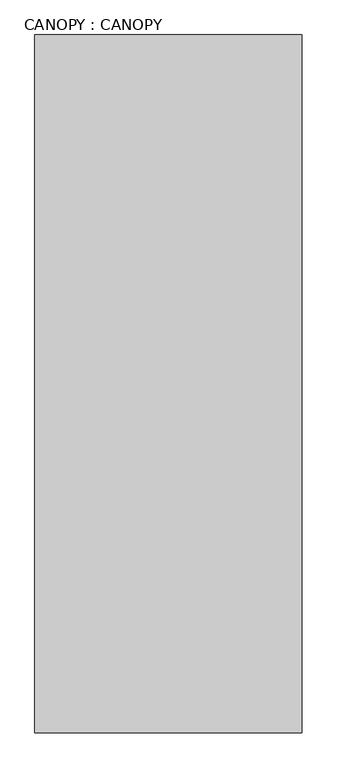
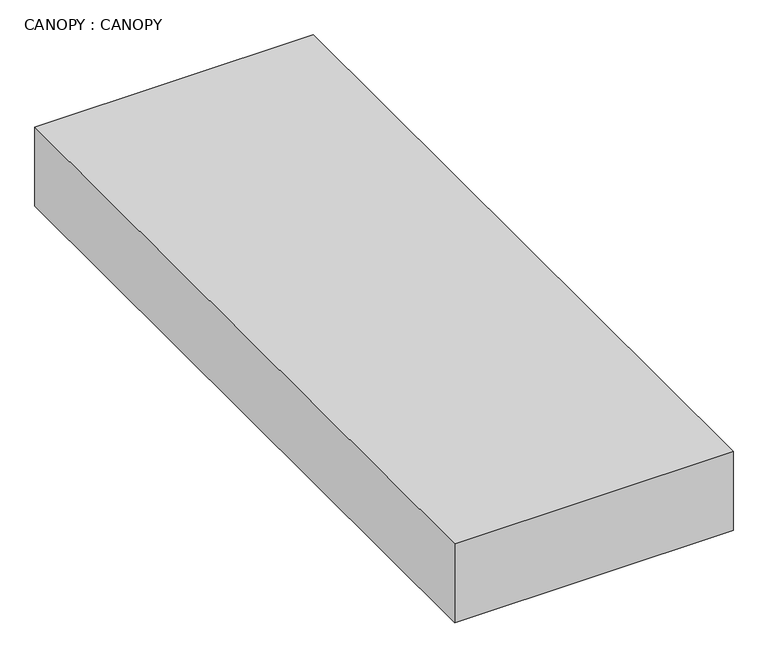
"""IFC4 building model written with IfcOpenShell, lengths in millimetres: proxy geometry, CANOPY : CANOPY."""

from ifc_helpers import new_model, si_unit, frame, origin, place, context, project, spatial, polyline, outline, extrude, source, transform, mapped, element, save


def canopy_canopy_9b852544(model_context):
    return source(origin(), model_context, "Body", "SweptSolid", [
        extrude(outline(polyline([(51934.0, 32404.5208589), (51934.0, 29794.5208589), (50934.0, 29794.5208589), (50934.0, 32404.5208589), (51934.0, 32404.5208589)])), frame((0.0, 0.0, 2904.9720055), z_axis=(0.0, 0.0, 1.0), x_axis=(1.0, 0.0, 0.0)), (0.0, 0.0, 1.0), 300.0),
    ])


if __name__ == "__main__":
    model = new_model("IFC4")
    model_context = context("Model", 3, world=origin())
    ifc_project = project(units=[si_unit("LENGTHUNIT", "METRE", prefix="MILLI")], contexts=[model_context])
    site = spatial("IfcSite", under=ifc_project)
    building = spatial("IfcBuilding", under=site)
    placement = place(None, origin())
    canopy_canopy_shape = canopy_canopy_9b852544(model_context)
    element("IfcBuildingElementProxy", 1, Name="CANOPY : CANOPY", ObjectType="CANOPY : CANOPY", at=placement, inside=building, context=model_context, shape_type="MappedRepresentation", body=[
        mapped(canopy_canopy_shape, transform((0.0, 0.0, 0.0), x_axis=(1.0, 0.0, 0.0), y_axis=(0.0, 1.0, 0.0), z_axis=(0.0, 0.0, 1.0))),
    ])
    save(model, "model.ifc")
